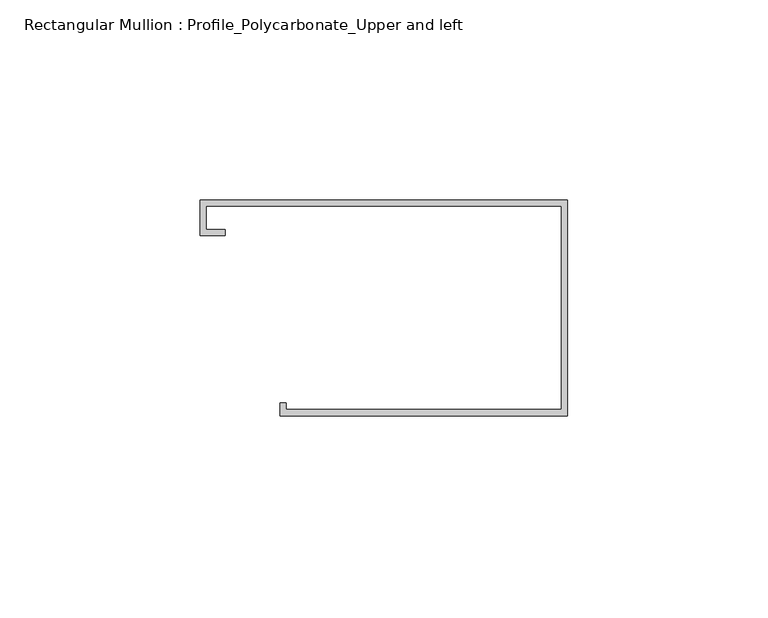
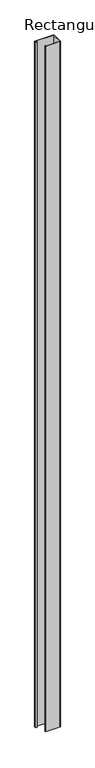
"""IFC4 building model written with IfcOpenShell, lengths in millimetres: member geometry, Rectangular Mullion : Profile_Polycarbonate_Upper and left."""

from ifc_helpers import new_model, si_unit, frame, origin, place, context, project, spatial, polyline, outline, extrude, source, transform, mapped, element, save


def rectangular_mullion_profile_polycarbonate_upper_and_left_5f3c44e9(model_context):
    return source(origin(), model_context, "Body", "SweptSolid", [
        extrude(outline(polyline([(0.0, 28.984575), (0.0, -25.015825), (-71.9836, -25.015825), (-71.9836, -21.840825), (-70.3961, -21.840825), (-70.3961, -23.428325), (-1.5875, -23.428325), (-1.5875, 27.397075), (-90.4113, 27.397075), (-90.4113, 21.580475), (-85.6488, 21.580475), (-85.6488, 19.992975), (-91.9988, 19.992975), (-91.9988, 28.984575), (0.0, 28.984575)])), frame((0.0, 0.0, -3475.3898378), z_axis=(0.0, 0.0, 1.0), x_axis=(1.0, 0.0, 0.0)), (0.0, 0.0, 1.0), 3475.3898378),
    ])


if __name__ == "__main__":
    model = new_model("IFC4")
    model_context = context("Model", 3, world=origin())
    ifc_project = project(units=[si_unit("LENGTHUNIT", "METRE", prefix="MILLI")], contexts=[model_context])
    site = spatial("IfcSite", under=ifc_project)
    building = spatial("IfcBuilding", under=site)
    placement = place(None, origin())
    rectangular_mullion_profile_polycarbonate_upper_and_left_shape = rectangular_mullion_profile_polycarbonate_upper_and_left_5f3c44e9(model_context)
    element("IfcMember", 1, ObjectType="Rectangular Mullion : Profile_Polycarbonate_Upper and left", at=placement, inside=building, context=model_context, shape_type="MappedRepresentation", body=[
        mapped(rectangular_mullion_profile_polycarbonate_upper_and_left_shape, transform((0.0, 0.0, 0.0), x_axis=(1.0, 0.0, 0.0), y_axis=(0.0, 1.0, 0.0), z_axis=(0.0, 0.0, 1.0))),
    ])
    save(model, "model.ifc")

# Revit data of these elements
# Type "Rectangular Mullion : Profile_Polycarbonate_Upper and left"
#   built-in parameter 1007322 = 0.177167 (stored number, unit not read)
#   built-in parameter 1007321 = 0.00520833 (stored number, unit not read)
#   built-in parameter 1007320 = 0 (stored number, unit not read)
